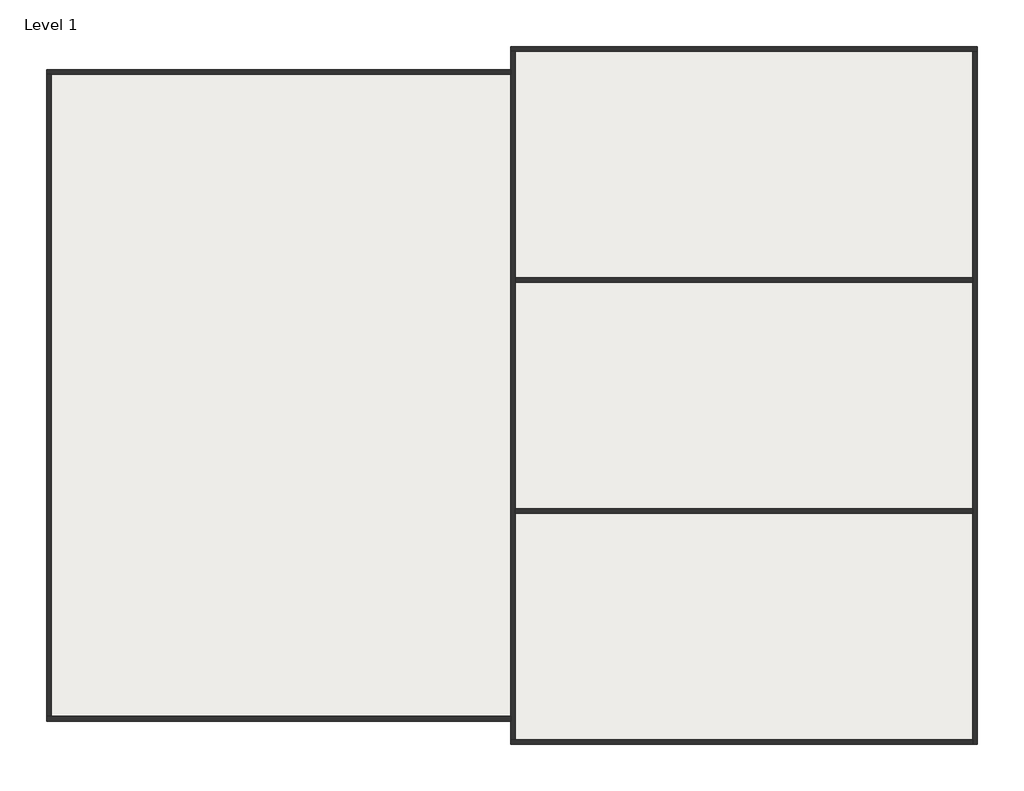
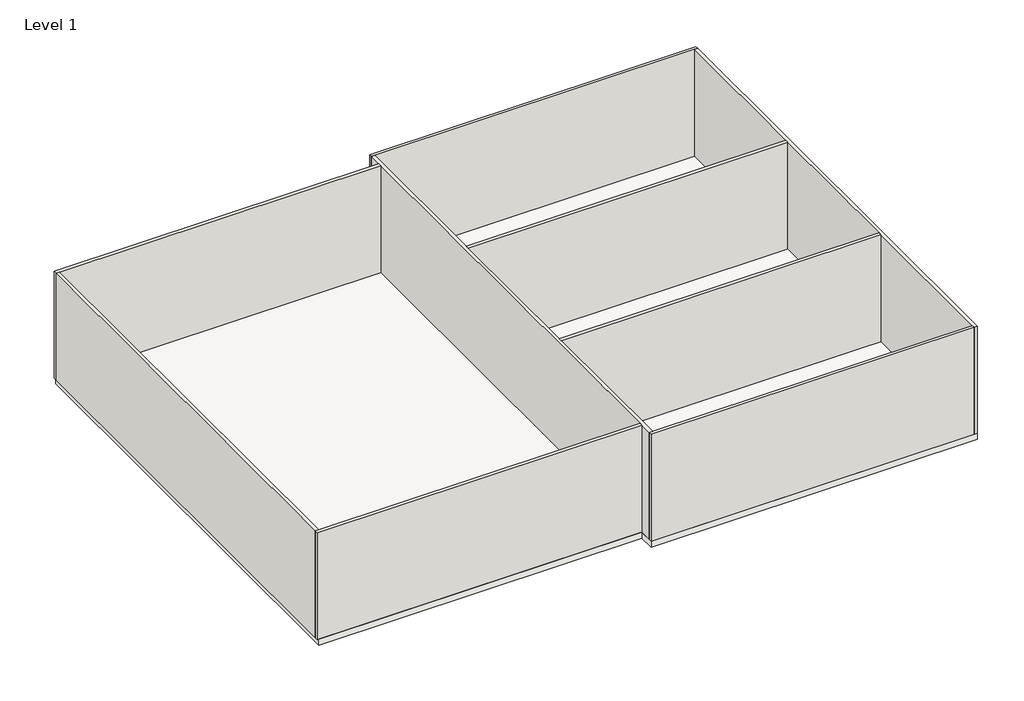
# One storey: 9 walls, 1 slab.
"""IFC4 building model written with IfcOpenShell, lengths in millimetres."""

from ifc_helpers import new_model, si_unit, frame, origin, origin_with_axes, place, context, project, spatial, polyline, outline, extrude, faceted_brep, element, save

model = new_model("IFC4")

# Units and contexts
model_context = context("Model", 3, world=origin())
ifc_project = project(units=[si_unit("LENGTHUNIT", "METRE", prefix="MILLI")], contexts=[model_context])

# Site, building, storey
site = spatial("IfcSite", under=ifc_project)
building = spatial("IfcBuilding", under=site)
storey = spatial("IfcBuildingStorey", under=building, Name="Level 1", Elevation=0.0)

# Slab
placement = place(None, origin())
element("IfcSlab", 1, ObjectType="Generic Floor - 400mm", at=placement, inside=storey, context=model_context, shape_type="SweptSolid", body=[
    extrude(outline(polyline([(15961.6453008, 15932.1645221), (15961.6453008, 16932.1645221), (36161.6453008, 16932.1645221), (36161.6453008, -13267.8354779), (15961.6453008, -13267.8354779), (15961.6453008, -12267.8354779), (-4038.3546992, -12267.8354779), (-4038.3546992, 15932.1645221), (15961.6453008, 15932.1645221)])), frame((0.0, 0.0, -400.0), z_axis=(0.0, 0.0, 1.0), x_axis=(1.0, 0.0, 0.0)), (0.0, 0.0, 1.0), 400.0),
])

# Walls
element("IfcWall", 2, ObjectType="Generic - 200mm", at=placement, inside=storey, context=model_context, shape_type="SweptSolid", body=[
    extrude(outline(polyline([(16161.6453008, 6932.1645221), (35961.6453008, 6932.1645221), (35961.6453008, 6732.1645221), (16161.6453008, 6732.1645221), (16161.6453008, 6932.1645221)])), origin_with_axes(), (0.0, 0.0, 1.0), 7000.0),
])
element("IfcWall", 3, ObjectType="Generic - 200mm", at=placement, inside=storey, context=model_context, shape_type="SweptSolid", body=[
    extrude(outline(polyline([(16161.6453008, -3067.8354779), (35961.6453008, -3067.8354779), (35961.6453008, -3267.8354779), (16161.6453008, -3267.8354779), (16161.6453008, -3067.8354779)])), origin_with_axes(), (0.0, 0.0, 1.0), 7000.0),
])
element("IfcWall", 4, ObjectType="Generic - 200mm", at=placement, inside=storey, context=model_context, shape_type="Brep", body=[
    faceted_brep([(16161.6453008, -13067.8354779, 0.0), (16161.6453008, -3267.8354779, 0.0), (16161.6453008, -3067.8354779, 0.0), (16161.6453008, 6732.1645221, 0.0), (16161.6453008, 6932.1645221, 0.0), (16161.6453008, 16732.1645221, 0.0), (16161.6453008, 16732.1645221, 7000.0), (16161.6453008, 6932.1645221, 7000.0), (16161.6453008, 6732.1645221, 7000.0), (16161.6453008, -3067.8354779, 7000.0), (16161.6453008, -3267.8354779, 7000.0), (16161.6453008, -13067.8354779, 7000.0), (15961.6453008, -13067.8354779, 0.0), (15961.6453008, -13067.8354779, 7000.0), (15961.6453008, -12267.8354779, 7000.0), (15961.6453008, -12067.8354779, 7000.0), (15961.6453008, 15732.1645221, 7000.0), (15961.6453008, 15932.1645221, 7000.0), (15961.6453008, 16732.1645221, 7000.0), (15961.6453008, 16732.1645221, 0.0), (15961.6453008, 15932.1645221, 0.0), (15961.6453008, 15732.1645221, 0.0), (15961.6453008, -12067.8354779, 0.0), (15961.6453008, -12267.8354779, 0.0)], [[[0, 1, 2, 3, 4, 5, 6, 7, 8, 9, 10, 11]], [[12, 13, 14, 15, 16, 17, 18, 19, 20, 21, 22, 23]], [[5, 4, 3, 2, 1, 0, 12, 23, 22, 21, 20, 19]], [[11, 10, 9, 8, 7, 6, 18, 17, 16, 15, 14, 13]], [[0, 11, 13, 12]], [[6, 5, 19, 18]]]),
])
element("IfcWall", 5, ObjectType="curtain wall - 200mm", at=placement, inside=storey, context=model_context, shape_type="Brep", body=[
    faceted_brep([(-4138.8546992, 15732.1645221, 0.0), (-3938.8546992, 15732.1645221, 0.0), (15961.6453008, 15732.1645221, 0.0), (15961.6453008, 15732.1645221, 7000.0), (-3938.8546992, 15732.1645221, 7000.0), (-4138.8546992, 15732.1645221, 7000.0), (-4138.8546992, 15932.1645221, 0.0), (-4138.8546992, 15932.1645221, 7000.0), (15961.6453008, 15932.1645221, 7000.0), (15961.6453008, 15932.1645221, 0.0)], [[[0, 1, 2, 3, 4, 5]], [[6, 7, 8, 9]], [[2, 1, 0, 6, 9]], [[5, 4, 3, 8, 7]], [[0, 5, 7, 6]], [[3, 2, 9, 8]]]),
])
element("IfcWall", 6, ObjectType="curtain wall - 200mm", at=placement, inside=storey, context=model_context, shape_type="Brep", body=[
    faceted_brep([(15961.6453008, 16732.1645221, 0.0), (16161.6453008, 16732.1645221, 0.0), (35961.6453008, 16732.1645221, 0.0), (36161.6453008, 16732.1645221, 0.0), (36161.6453008, 16732.1645221, 7000.0), (35961.6453008, 16732.1645221, 7000.0), (16161.6453008, 16732.1645221, 7000.0), (15961.6453008, 16732.1645221, 7000.0), (15961.6453008, 16932.1645221, 0.0), (15961.6453008, 16932.1645221, 7000.0), (36161.6453008, 16932.1645221, 7000.0), (36161.6453008, 16932.1645221, 0.0)], [[[0, 1, 2, 3, 4, 5, 6, 7]], [[8, 9, 10, 11]], [[3, 2, 1, 0, 8, 11]], [[7, 6, 5, 4, 10, 9]], [[4, 3, 11, 10]], [[0, 7, 9, 8]]]),
])
element("IfcWall", 7, ObjectType="curtain wall - 200mm", at=placement, inside=storey, context=model_context, shape_type="Brep", body=[
    faceted_brep([(35961.6453008, 16732.1645221, 0.0), (35961.6453008, 6932.1645221, 0.0), (35961.6453008, 6732.1645221, 0.0), (35961.6453008, -3067.8354779, 0.0), (35961.6453008, -3267.8354779, 0.0), (35961.6453008, -13067.8354779, 0.0), (35961.6453008, -13267.8354779, 0.0), (35961.6453008, -13267.8354779, 7000.0), (35961.6453008, -13067.8354779, 7000.0), (35961.6453008, -3267.8354779, 7000.0), (35961.6453008, -3067.8354779, 7000.0), (35961.6453008, 6732.1645221, 7000.0), (35961.6453008, 6932.1645221, 7000.0), (35961.6453008, 16732.1645221, 7000.0), (36161.6453008, 16732.1645221, 0.0), (36161.6453008, 16732.1645221, 7000.0), (36161.6453008, -13267.8354779, 7000.0), (36161.6453008, -13267.8354779, 0.0)], [[[0, 1, 2, 3, 4, 5, 6, 7, 8, 9, 10, 11, 12, 13]], [[14, 15, 16, 17]], [[6, 5, 4, 3, 2, 1, 0, 14, 17]], [[13, 12, 11, 10, 9, 8, 7, 16, 15]], [[0, 13, 15, 14]], [[7, 6, 17, 16]]]),
])
element("IfcWall", 8, ObjectType="curtain wall - 200mm", at=placement, inside=storey, context=model_context, shape_type="Brep", body=[
    faceted_brep([(35961.6453008, -13067.8354779, 0.0), (16161.6453008, -13067.8354779, 0.0), (15961.6453008, -13067.8354779, 0.0), (15961.6453008, -13067.8354779, 7000.0), (16161.6453008, -13067.8354779, 7000.0), (35961.6453008, -13067.8354779, 7000.0), (35961.6453008, -13267.8354779, 0.0), (35961.6453008, -13267.8354779, 7000.0), (15961.6453008, -13267.8354779, 7000.0), (15961.6453008, -13267.8354779, 0.0)], [[[0, 1, 2, 3, 4, 5]], [[6, 7, 8, 9]], [[2, 1, 0, 6, 9]], [[5, 4, 3, 8, 7]], [[0, 5, 7, 6]], [[3, 2, 9, 8]]]),
])
element("IfcWall", 9, ObjectType="curtain wall - 200mm", at=placement, inside=storey, context=model_context, shape_type="Brep", body=[
    faceted_brep([(15961.6453008, -12067.8354779, 0.0), (-3938.8546992, -12067.8354779, 0.0), (-4138.8546992, -12067.8354779, 0.0), (-4138.8546992, -12067.8354779, 7000.0), (-3938.8546992, -12067.8354779, 7000.0), (15961.6453008, -12067.8354779, 7000.0), (15961.6453008, -12267.8354779, 0.0), (15961.6453008, -12267.8354779, 7000.0), (-4138.8546992, -12267.8354779, 7000.0), (-4138.8546992, -12267.8354779, 0.0)], [[[0, 1, 2, 3, 4, 5]], [[6, 7, 8, 9]], [[2, 1, 0, 6, 9]], [[5, 4, 3, 8, 7]], [[0, 5, 7, 6]], [[3, 2, 9, 8]]]),
])
element("IfcWall", 10, ObjectType="curtain wall - 200mm", at=placement, inside=storey, context=model_context, shape_type="SweptSolid", body=[
    extrude(outline(polyline([(-3938.8546992, 15732.1645221), (-3938.8546992, -12067.8354779), (-4138.8546992, -12067.8354779), (-4138.8546992, 15732.1645221), (-3938.8546992, 15732.1645221)])), origin_with_axes(), (0.0, 0.0, 1.0), 7000.0),
])

save(model, "model.ifc")

# Revit data of these elements
# Project information
#   Project Issue Date = "Issue Date"
#   Project Status = "Project Status"
#   Client Name = "Owner"
#   Project Address = "Enter address here"
#   Project Name = "Project Name"
#   Project Number = "Project Number"
# Grids (mm)
#   "B": line (-13464.174, 15932.165) -> (41880.766, 15932.165)
#   "1": line (-4138.855, -18194.081) -> (-4138.855, 22725.592)
#   "2": line (16061.645, -19435.057) -> (16061.645, 22725.592)
#   "3": line (36161.645, -19435.057) -> (36161.645, 22725.592)
#   "A": line (-13464.174, -12267.835) -> (41880.766, -12267.835)
# Type "Generic Floor - 400mm"
#   Function = 0
#   Layers, outside or top first: 400 mm no material (function 1)
# Type "Generic - 200mm"
#   Layers, outside or top first: 200 mm no material (function 1)
# Type "curtain wall - 200mm"
#   Layers, outside or top first: 200 mm "Glass, Clear Glazing" (function 1)
# Element 1 (IfcSlab, "Generic Floor - 400mm")
#   Height Offset From Level = 0 mm
#   Phase Created = New Construction
#   Materials on its faces: "Default Floor"
# Elements 2, 3, 4 (IfcWall, "Generic - 200mm")
#   Top Offset = 0 mm
#   Base Offset = 0 mm
#   wall height = 7000 mm
#   Phase Created = New Construction
#   Base Constraint = Level 1
#   Top Constraint = Level 2
#   Materials on its faces: "Default Wall"
# Elements 5, 7, 9, 10 (IfcWall, "curtain wall - 200mm")
#   Top Offset = 0 mm
#   Base Offset = 0 mm
#   wall height = 7000 mm
#   Phase Created = New Construction
#   Base Constraint = Level 1
#   Top Constraint = Level 2
#   Materials on its faces: "Glass, Clear Glazing"
# Elements 6, 8 (IfcWall, "curtain wall - 200mm")
#   Top Offset = 0 mm
#   Base Offset = 0 mm
#   wall height = 7000 mm
#   Phase Created = New Construction
#   Base Constraint = Level 1
#   Top Constraint = Level 2
#   Materials on its faces: "Glass, Clear Glazing", "Default Wall"
# Materials
#   "Glass, Clear Glazing": class "Glass", colour RGB 0 128 192, transparency 0.75, Description = "Clear glazing", Cost = 0
#   "Default Floor": class "Miscellaneous", colour RGB 127 127 127, transparency 0, Cost = 0
#   "Default Wall": class "Miscellaneous", colour RGB 128 128 128, transparency 0, Cost = 0
# Room at (5886.89, 1766.376) mm, phase "New Construction", upper level "Level 2", upper offset 0 mm, lower offset 0 mm
#   Number = "1"
#   Name = "Room"
# Room at (26105.253, 11567.522) mm, phase "New Construction", upper level "Level 2", upper offset 0 mm, lower offset 0 mm
#   Number = "2"
#   Name = "Room"
# Room at (25993.24, 1934.396) mm, phase "New Construction", upper level "Level 2", upper offset 0 mm, lower offset 0 mm
#   Number = "3"
#   Name = "Room"
# Room at (26161.26, -8146.782) mm, phase "New Construction", upper level "Level 2", upper offset 0 mm, lower offset 0 mm
#   Number = "4"
#   Name = "Room"
